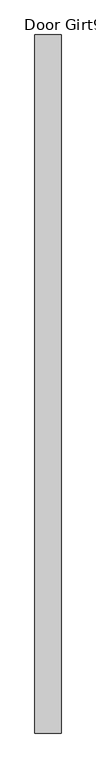
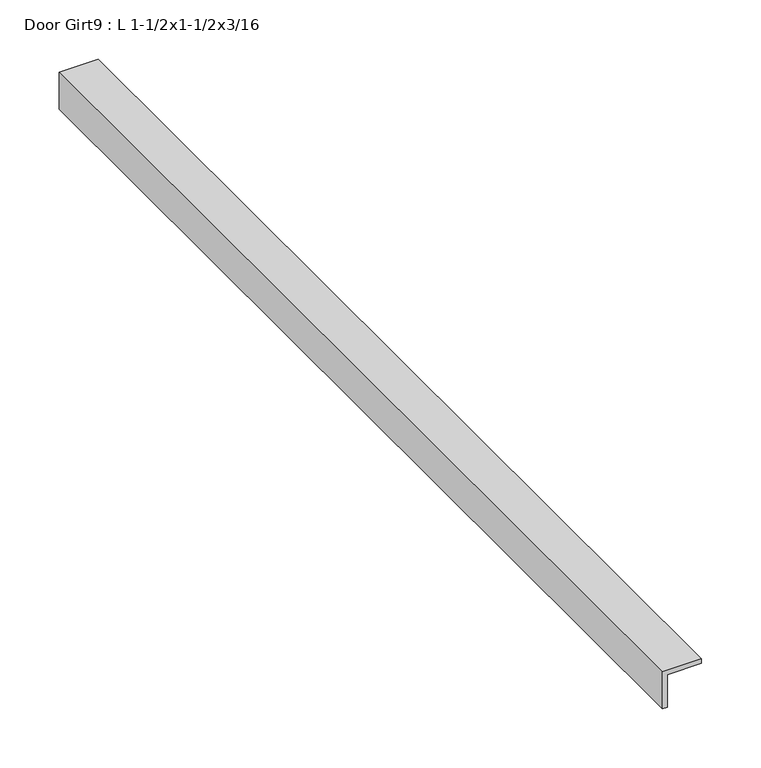
"""IFC4 building model written with IfcOpenShell, lengths in millimetres: proxy geometry, Door Girt9 : L 1-1/2x1-1/2x3/16."""

from ifc_helpers import new_model, si_unit, frame, origin, place, context, project, spatial, polyline, outline, extrude, source, transform, mapped, element, save


def door_girt9_l_1_1_2x1_1_2x3_16_7802d8c0(model_context):
    return source(origin(), model_context, "Body", "SweptSolid", [
        extrude(outline(polyline([(1625.6, 587403.9934739), (1625.6, 587365.8934739), (1587.5, 587365.8934739), (1587.5, 587370.6559739), (1620.8375, 587370.6559739), (1620.8375, 587403.9934739), (1625.6, 587403.9934739)])), frame((0.0, -535163.4663841, 0.0), z_axis=(0.0, 1.0, 0.0), x_axis=(0.0, 0.0, 1.0)), (0.0, 0.0, 1.0), 1017.5875),
    ])


if __name__ == "__main__":
    model = new_model("IFC4")
    model_context = context("Model", 3, world=origin())
    ifc_project = project(units=[si_unit("LENGTHUNIT", "METRE", prefix="MILLI")], contexts=[model_context])
    site = spatial("IfcSite", under=ifc_project)
    building = spatial("IfcBuilding", under=site)
    placement = place(None, origin())
    door_girt9_l_1_1_2x1_1_2x3_16_shape = door_girt9_l_1_1_2x1_1_2x3_16_7802d8c0(model_context)
    element("IfcBuildingElementProxy", 1, Name="Door Girt9 : L 1-1/2x1-1/2x3/16", ObjectType="Door Girt9 : L 1-1/2x1-1/2x3/16", at=placement, inside=building, context=model_context, shape_type="MappedRepresentation", body=[
        mapped(door_girt9_l_1_1_2x1_1_2x3_16_shape, transform((0.0, 0.0, 0.0), x_axis=(1.0, 0.0, 0.0), y_axis=(0.0, 1.0, 0.0), z_axis=(0.0, 0.0, 1.0))),
    ])
    save(model, "model.ifc")

# Revit data of these elements
# Element 1 (IfcBuildingElementProxy, "Door Girt9 : L 1-1/2x1-1/2x3/16")
#   Materials on its faces: "1-1/2\"X1-1/2\" GALV. STL L"
# Materials
#   "1-1/2\"X1-1/2\" GALV. STL L": class "Generic", colour RGB 211 211 207, transparency 0, Cost = 0
